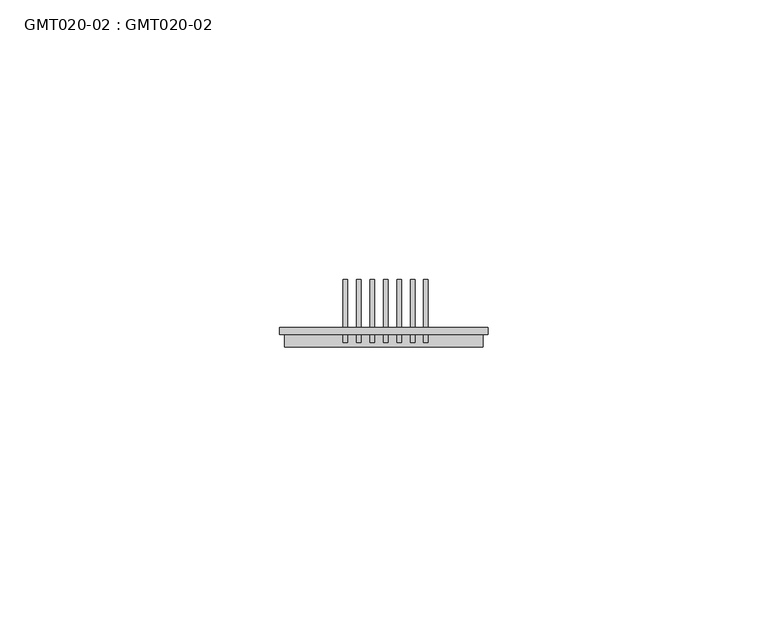
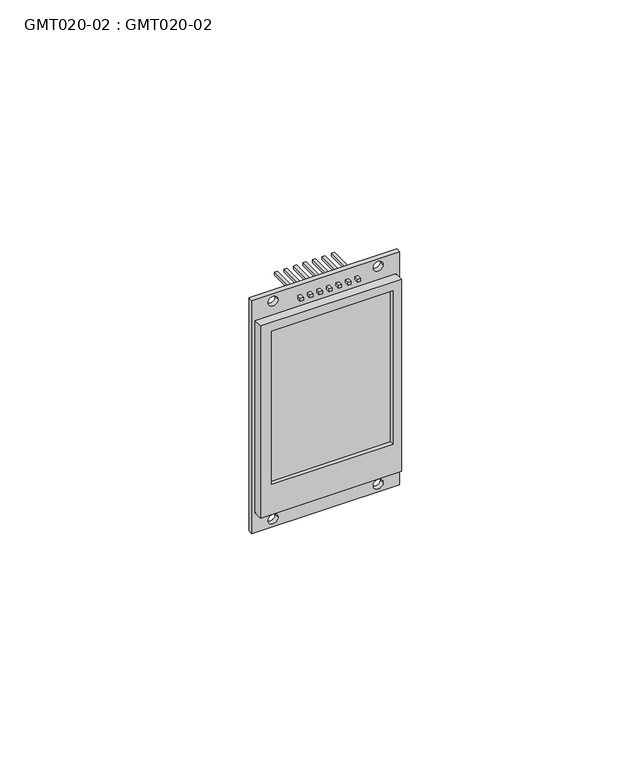
"""IFC4 building model written with IfcOpenShell, lengths in millimetres: furniture geometry, GMT020-02 : GMT020-02."""

from ifc_helpers import new_model, si_unit, frame, origin, place, context, project, spatial, polyline, circle_curve, outline, extrude, source, transform, mapped, element, save
from ifc_brep_helpers import plane_surface, revolved_surface, advanced_brep


def gmt020_02_gmt020_02_ca843257(model_context):
    return source(origin(), model_context, "Body", "SolidModel", [
        advanced_brep(
        [(18.3, -32.2, 62.0), (18.3, -31.0, 62.0), (-19.0, -31.0, 62.0), (-19.0, -32.2, 62.0), (18.3, -32.2, 0.0), (-19.0, -32.2, 0.0), (-19.0, -31.0, 0.0), (18.3, -31.0, 0.0), (-14.85, -31.0, 60.0), (-12.35, -31.0, 60.0), (-14.85, -31.0, 2.0), (-12.35, -31.0, 2.0), (14.15, -31.0, 60.0), (11.65, -31.0, 60.0), (14.15, -31.0, 2.0), (11.65, -31.0, 2.0), (-18.1, -32.2, 56.4), (17.4, -32.2, 56.4), (17.4, -32.2, 5.2), (-18.1, -32.2, 5.2), (-12.35, -32.2, 60.0), (-14.85, -32.2, 60.0), (-12.35, -32.2, 2.0), (-14.85, -32.2, 2.0), (11.65, -32.2, 60.0), (14.15, -32.2, 60.0), (11.65, -32.2, 2.0), (14.15, -32.2, 2.0), (17.4, -34.4693991, 56.4), (-18.1, -34.4693991, 56.4), (17.4, -34.4693991, 5.2), (-18.1, -34.4693991, 5.2), (-15.3, -34.4693991, 54.0), (15.3, -34.4693991, 54.0), (15.3, -34.4693991, 13.2), (-15.3, -34.4693991, 13.2), (-15.3, -33.4693991, 54.0), (15.3, -33.4693991, 54.0), (15.3, -33.4693991, 13.2), (-15.3, -33.4693991, 13.2)],
        [
            (0, 1),
            (1, 2),
            (2, 3),
            (3, 0),
            (4, 5),
            (5, 6),
            (6, 7),
            (7, 4),
            (0, 4),
            (7, 1),
            (6, 2),
            (8, 9, circle_curve(frame((-13.6, -31.0, 60.0), z_axis=(0.0, -1.0, 0.0), x_axis=(1.0, 0.0, 0.0)), 1.25)),
            (9, 8, circle_curve(frame((-13.6, -31.0, 60.0), z_axis=(0.0, -1.0, 0.0), x_axis=(1.0, 0.0, 0.0)), 1.25)),
            (10, 11, circle_curve(frame((-13.6, -31.0, 2.0), z_axis=(0.0, -1.0, 0.0), x_axis=(1.0, 0.0, 0.0)), 1.25)),
            (11, 10, circle_curve(frame((-13.6, -31.0, 2.0), z_axis=(0.0, -1.0, 0.0), x_axis=(1.0, 0.0, 0.0)), 1.25)),
            (12, 13, circle_curve(frame((12.9, -31.0, 60.0), z_axis=(0.0, -1.0, 0.0), x_axis=(-1.0, 0.0, 0.0)), 1.25)),
            (13, 12, circle_curve(frame((12.9, -31.0, 60.0), z_axis=(0.0, -1.0, 0.0), x_axis=(-1.0, 0.0, 0.0)), 1.25)),
            (14, 15, circle_curve(frame((12.9, -31.0, 2.0), z_axis=(0.0, -1.0, 0.0), x_axis=(-1.0, 0.0, 0.0)), 1.25)),
            (15, 14, circle_curve(frame((12.9, -31.0, 2.0), z_axis=(0.0, -1.0, 0.0), x_axis=(-1.0, 0.0, 0.0)), 1.25)),
            (5, 3),
            (16, 17),
            (17, 18),
            (18, 19),
            (19, 16),
            (20, 21, circle_curve(frame((-13.6, -32.2, 60.0), z_axis=(0.0, 1.0, 0.0), x_axis=(1.0, 0.0, 0.0)), 1.25)),
            (21, 20, circle_curve(frame((-13.6, -32.2, 60.0), z_axis=(0.0, 1.0, 0.0), x_axis=(1.0, 0.0, 0.0)), 1.25)),
            (22, 23, circle_curve(frame((-13.6, -32.2, 2.0), z_axis=(0.0, 1.0, 0.0), x_axis=(1.0, 0.0, 0.0)), 1.25)),
            (23, 22, circle_curve(frame((-13.6, -32.2, 2.0), z_axis=(0.0, 1.0, 0.0), x_axis=(1.0, 0.0, 0.0)), 1.25)),
            (24, 25, circle_curve(frame((12.9, -32.2, 60.0), z_axis=(0.0, 1.0, 0.0), x_axis=(-1.0, 0.0, 0.0)), 1.25)),
            (25, 24, circle_curve(frame((12.9, -32.2, 60.0), z_axis=(0.0, 1.0, 0.0), x_axis=(-1.0, 0.0, 0.0)), 1.25)),
            (26, 27, circle_curve(frame((12.9, -32.2, 2.0), z_axis=(0.0, 1.0, 0.0), x_axis=(-1.0, 0.0, 0.0)), 1.25)),
            (27, 26, circle_curve(frame((12.9, -32.2, 2.0), z_axis=(0.0, 1.0, 0.0), x_axis=(-1.0, 0.0, 0.0)), 1.25)),
            (28, 17),
            (16, 29),
            (29, 28),
            (30, 31),
            (31, 19),
            (18, 30),
            (28, 30),
            (31, 29),
            (32, 33),
            (33, 34),
            (34, 35),
            (35, 32),
            (8, 21),
            (20, 9),
            (10, 23),
            (22, 11),
            (32, 36),
            (36, 37),
            (37, 33),
            (34, 38),
            (38, 39),
            (39, 35),
            (37, 38),
            (36, 39),
            (12, 25),
            (24, 13),
            (14, 27),
            (26, 15),
        ],
        [
            plane_surface(frame((18.3, -32.2, 62.0), z_axis=(0.0, 0.0, 1.0), x_axis=(0.0, 1.0, 0.0))),
            plane_surface(frame((18.3, -32.2, 0.0), z_axis=(0.0, 0.0, -1.0), x_axis=(0.0, -1.0, 0.0))),
            plane_surface(frame((18.3, -32.2, 62.0), z_axis=(1.0, 0.0, 0.0), x_axis=(0.0, 0.0, -1.0))),
            plane_surface(frame((18.3, -31.0, 62.0), z_axis=(0.0, 1.0, 0.0), x_axis=(0.0, 0.0, -1.0))),
            plane_surface(frame((-19.0, -31.0, 62.0), z_axis=(-1.0, 0.0, 0.0), x_axis=(0.0, 0.0, -1.0))),
            plane_surface(frame((-19.0, -32.2, 62.0), z_axis=(0.0, -1.0, 0.0), x_axis=(0.0, 0.0, -1.0))),
            plane_surface(frame((17.4, -33.4693991, 56.4), z_axis=(0.0, 0.0, 1.0), x_axis=(0.0, 1.0, 0.0))),
            plane_surface(frame((17.4, -33.4693991, 5.2), z_axis=(0.0, 0.0, -1.0), x_axis=(0.0, -1.0, 0.0))),
            plane_surface(frame((17.4, -34.4693991, 56.4), z_axis=(1.0, 0.0, 0.0), x_axis=(0.0, 0.0, -1.0))),
            plane_surface(frame((-18.1, -32.2693991, 56.4), z_axis=(-1.0, 0.0, 0.0), x_axis=(0.0, 0.0, -1.0))),
            plane_surface(frame((-18.1, -34.4693991, 56.4), z_axis=(0.0, -1.0, 0.0), x_axis=(0.0, 0.0, -1.0))),
            revolved_surface(polyline([(-12.35, -32.2, 60.0), (-12.35, -31.0, 60.0)]), (-13.6, -28.9796632, 60.0), (0.0, -1.0, 0.0)),
            revolved_surface(polyline([(-12.35, -32.2, 2.0), (-12.35, -31.0, 2.0)]), (-13.6, -28.9796632, 2.0), (0.0, -1.0, 0.0)),
            plane_surface(frame((15.3, -34.4, 54.0), z_axis=(0.0, 0.0, -1.0), x_axis=(0.0, 1.0, 0.0))),
            plane_surface(frame((15.3, -34.4, 13.2), z_axis=(0.0, 0.0, 1.0), x_axis=(0.0, -1.0, 0.0))),
            plane_surface(frame((15.3, -34.4693991, 54.0), z_axis=(-1.0, 0.0, 0.0), x_axis=(0.0, 0.0, -1.0))),
            plane_surface(frame((15.3, -33.4693991, 54.0), z_axis=(0.0, -1.0, 0.0), x_axis=(0.0, 0.0, -1.0))),
            plane_surface(frame((-15.3, -33.4693991, 54.0), z_axis=(1.0, 0.0, 0.0), x_axis=(0.0, 0.0, -1.0))),
            revolved_surface(polyline([(11.65, -32.2, 60.0), (11.65, -31.0, 60.0)]), (12.9, -31.0, 60.0), (0.0, -1.0, 0.0)),
            revolved_surface(polyline([(11.65, -32.2, 2.0), (11.65, -31.0, 2.0)]), (12.9, -31.0, 2.0), (0.0, -1.0, 0.0)),
        ],
        [
            (0, [[1, 2, 3, 4]]),
            (1, [[5, 6, 7, 8]]),
            (2, [[-1, 9, -8, 10]]),
            (3, [[-2, -10, -7, 11], [12, 13], [14, 15], [16, 17], [18, 19]]),
            (4, [[-3, -11, -6, 20]]),
            (5, [[-4, -20, -5, -9], [21, 22, 23, 24], [25, 26], [27, 28], [29, 30], [31, 32]]),
            (6, [[33, -21, 34, 35]]),
            (7, [[36, 37, -23, 38]]),
            (8, [[-33, 39, -38, -22]]),
            (9, [[-34, -24, -37, 40]]),
            (10, [[-35, -40, -36, -39], [41, 42, 43, 44]]),
            (11, [[45, -25, 46, -12]]),
            (11, [[-45, -13, -46, -26]]),
            (12, [[47, -27, 48, -14]]),
            (12, [[-47, -15, -48, -28]]),
            (13, [[49, 50, 51, -41]]),
            (14, [[52, 53, 54, -43]]),
            (15, [[-51, 55, -52, -42]]),
            (16, [[-50, 56, -53, -55]]),
            (17, [[-49, -44, -54, -56]]),
            (18, [[57, -29, 58, -16]]),
            (18, [[-57, -17, -58, -30]]),
            (19, [[59, -31, 60, -18]]),
            (19, [[-59, -19, -60, -32]]),
        ],
    ),
        extrude(outline(polyline([(-7.6, -33.6693991), (-7.6, -22.3693991), (-6.8, -22.3693991), (-6.8, -33.6693991), (-7.6, -33.6693991)])), frame((0.0, 0.0, 58.8), z_axis=(0.0, 0.0, 1.0), x_axis=(1.0, 0.0, 0.0)), (0.0, 0.0, 1.0), 0.8),
        extrude(outline(polyline([(6.8, -33.6693991), (6.8, -22.3693991), (7.6, -22.3693991), (7.6, -33.6693991), (6.8, -33.6693991)])), frame((0.0, 0.0, 58.8), z_axis=(0.0, 0.0, 1.0), x_axis=(1.0, 0.0, 0.0)), (0.0, 0.0, 1.0), 0.8),
        extrude(outline(polyline([(4.4, -33.6693991), (4.4, -22.3693991), (5.2, -22.3693991), (5.2, -33.6693991), (4.4, -33.6693991)])), frame((0.0, 0.0, 58.8), z_axis=(0.0, 0.0, 1.0), x_axis=(1.0, 0.0, 0.0)), (0.0, 0.0, 1.0), 0.8),
        extrude(outline(polyline([(2.0, -33.6693991), (2.0, -22.3693991), (2.8, -22.3693991), (2.8, -33.6693991), (2.0, -33.6693991)])), frame((0.0, 0.0, 58.8), z_axis=(0.0, 0.0, 1.0), x_axis=(1.0, 0.0, 0.0)), (0.0, 0.0, 1.0), 0.8),
        extrude(outline(polyline([(-0.4, -33.6693991), (-0.4, -22.3693991), (0.4, -22.3693991), (0.4, -33.6693991), (-0.4, -33.6693991)])), frame((0.0, 0.0, 58.8), z_axis=(0.0, 0.0, 1.0), x_axis=(1.0, 0.0, 0.0)), (0.0, 0.0, 1.0), 0.8),
        extrude(outline(polyline([(-2.8, -33.6693991), (-2.8, -22.3693991), (-2.0, -22.3693991), (-2.0, -33.6693991), (-2.8, -33.6693991)])), frame((0.0, 0.0, 58.8), z_axis=(0.0, 0.0, 1.0), x_axis=(1.0, 0.0, 0.0)), (0.0, 0.0, 1.0), 0.8),
        extrude(outline(polyline([(-5.2, -33.6693991), (-5.2, -22.3693991), (-4.4, -22.3693991), (-4.4, -33.6693991), (-5.2, -33.6693991)])), frame((0.0, 0.0, 58.8), z_axis=(0.0, 0.0, 1.0), x_axis=(1.0, 0.0, 0.0)), (0.0, 0.0, 1.0), 0.8),
    ])


if __name__ == "__main__":
    model = new_model("IFC4")
    model_context = context("Model", 3, world=origin())
    ifc_project = project(units=[si_unit("LENGTHUNIT", "METRE", prefix="MILLI")], contexts=[model_context])
    site = spatial("IfcSite", under=ifc_project)
    building = spatial("IfcBuilding", under=site)
    placement = place(None, origin())
    gmt020_02_gmt020_02_shape = gmt020_02_gmt020_02_ca843257(model_context)
    element("IfcFurniture", 1, ObjectType="GMT020-02 : GMT020-02", at=placement, inside=building, context=model_context, shape_type="MappedRepresentation", body=[
        mapped(gmt020_02_gmt020_02_shape, transform((0.0, 0.0, 0.0), x_axis=(1.0, 0.0, 0.0), y_axis=(0.0, 1.0, 0.0), z_axis=(0.0, 0.0, 1.0))),
    ])
    save(model, "model.ifc")

# Revit data of these elements
# Type "GMT020-02 : GMT020-02"
#   Default Elevation = 0
# Element 1 (IfcFurniture, "GMT020-02 : GMT020-02")
#   Materials on its faces: ".TELA"
# Materials
#   ".TELA": class "Vidro", colour RGB 128 128 255, transparency 0.5, Cost = 0
